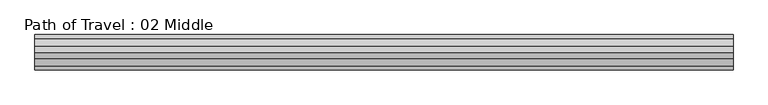
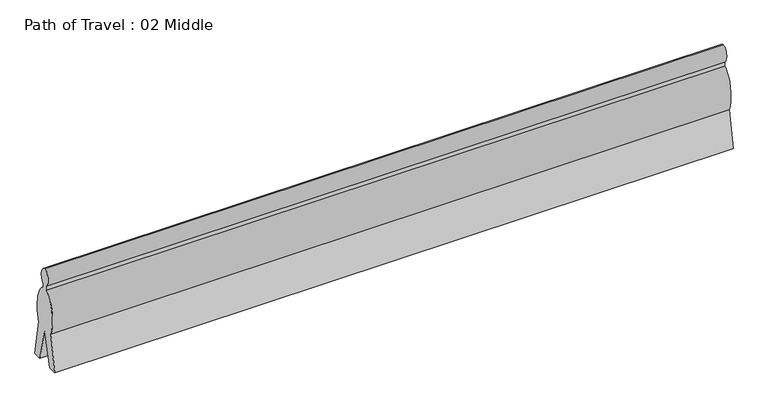
"""IFC4 building model written with IfcOpenShell, lengths in millimetres: proxy geometry, Path of Travel : 02 Middle."""

from ifc_helpers import new_model, si_unit, point, frame, origin, place, context, project, spatial, ellipse_curve, trimmed, source, transform, mapped, element, save
from ifc_brep_helpers import plane_surface, extruded_surface, advanced_brep


def path_of_travel_02_middle_84569f44(model_context):
    return source(origin(), model_context, "Body", "AdvancedBrep", [
        advanced_brep(
        [(227.5554837, 0.0, 1727.2), (227.5554837, 42.9018657, 1436.6534209), (227.5554837, 42.9018657, 1363.4763406), (227.5554837, 184.1186263, 643.4144547), (227.5554837, 297.5699544, 0.0), (227.5554837, 145.6574193, 0.0), (227.5554837, 0.0, 584.2), (227.5554837, -145.6574193, 0.0), (227.5554837, -297.5699544, 0.0), (227.5554837, -184.1186263, 643.4144547), (227.5554837, -42.9018657, 1363.4763406), (227.5554837, -42.9018657, 1436.6534209), (11987.6438615, 0.0, 1727.2), (11987.6438615, -42.9018657, 1436.6534209), (11987.6438615, -42.9018657, 1363.4763406), (11987.6438615, -184.1186263, 643.4144547), (11987.6438615, -297.5699544, 0.0), (11987.6438615, -145.6574193, 0.0), (11987.6438615, 0.0, 584.2), (11987.6438615, 145.6574193, 0.0), (11987.6438615, 297.5699544, 0.0), (11987.6438615, 184.1186263, 643.4144547), (11987.6438615, 42.9018657, 1363.4763406), (11987.6438615, 42.9018657, 1436.6534209)],
        [
            (0, 1, ellipse_curve(frame((227.5554837, 0.0, 1574.8), z_axis=(-1.0, 0.0, 0.0), x_axis=(0.0, 0.0, 1.0)), 152.4, 101.6)),
            (1, 2),
            (2, 3, ellipse_curve(frame((227.5554837, 0.0, 914.4), z_axis=(-1.0, 0.0, 0.0), x_axis=(0.0, 0.0, -1.0)), 457.2, 228.6)),
            (3, 4),
            (4, 5),
            (5, 6),
            (6, 7),
            (7, 8),
            (8, 9),
            (9, 10, ellipse_curve(frame((227.5554837, 0.0, 914.4), z_axis=(-1.0, 0.0, 0.0), x_axis=(0.0, 0.0, -1.0)), 457.2, 228.6)),
            (10, 11),
            (11, 0, ellipse_curve(frame((227.5554837, 0.0, 1574.8), z_axis=(-1.0, 0.0, 0.0), x_axis=(0.0, 0.0, 1.0)), 152.4, 101.6)),
            (12, 13, ellipse_curve(frame((11987.6438615, 0.0, 1574.8), z_axis=(1.0, 0.0, 0.0), x_axis=(0.0, 0.0, 1.0)), 152.4, 101.6)),
            (13, 14),
            (14, 15, ellipse_curve(frame((11987.6438615, 0.0, 914.4), z_axis=(1.0, 0.0, 0.0), x_axis=(0.0, 0.0, -1.0)), 457.2, 228.6)),
            (15, 16),
            (16, 17),
            (17, 18),
            (18, 19),
            (19, 20),
            (20, 21),
            (21, 22, ellipse_curve(frame((11987.6438615, 0.0, 914.4), z_axis=(1.0, 0.0, 0.0), x_axis=(0.0, 0.0, -1.0)), 457.2, 228.6)),
            (22, 23),
            (23, 12, ellipse_curve(frame((11987.6438615, 0.0, 1574.8), z_axis=(1.0, 0.0, 0.0), x_axis=(0.0, 0.0, 1.0)), 152.4, 101.6)),
            (0, 12),
            (23, 1),
            (22, 2),
            (21, 3),
            (20, 4),
            (19, 5),
            (18, 6),
            (17, 7),
            (16, 8),
            (15, 9),
            (14, 10),
            (13, 11),
        ],
        [
            plane_surface(frame((227.5554837, 0.0, 0.0), z_axis=(-1.0, 0.0, 0.0), x_axis=(0.0, 0.0, 1.0))),
            plane_surface(frame((11987.6438615, 0.0, 0.0), z_axis=(1.0, 0.0, 0.0), x_axis=(0.0, 0.0, 1.0))),
            extruded_surface(trimmed(ellipse_curve(frame((11987.6438615, 0.0, 1574.8), z_axis=(-1.0, 0.0, 0.0), x_axis=(0.0, 0.0, 1.0)), 152.4, 101.6), [point((11987.6438615, 0.0, 1727.2))], [point((11987.6438615, 42.9018657, 1436.6534209))], True, "CARTESIAN"), (-11760.0883778, 0.0, 0.0), 11760.0883778),
            plane_surface(frame((227.5554837, 42.9018657, 1436.6534209), z_axis=(0.0, 1.0, 0.0), x_axis=(1.0, 0.0, 0.0))),
            extruded_surface(trimmed(ellipse_curve(frame((11987.6438615, 0.0, 914.4), z_axis=(-1.0, 0.0, 0.0), x_axis=(0.0, 0.0, -1.0)), 457.2, 228.6), [point((11987.6438615, 42.9018657, 1363.4763406))], [point((11987.6438615, 184.1186263, 643.4144547))], True, "CARTESIAN"), (-11760.0883778, 0.0, 0.0), 11760.0883778),
            plane_surface(frame((227.5554837, 184.1186263, 643.4144547), z_axis=(0.0, 0.9848077530122078, 0.17364817766693205), x_axis=(1.0, 0.0, 0.0))),
            plane_surface(frame((227.5554837, 297.5699544, 0.0), z_axis=(0.0, 0.0, -1.0), x_axis=(1.0, 0.0, 0.0))),
            plane_surface(frame((227.5554837, 145.6574193, 0.0), z_axis=(0.0, -0.9702957262760199, -0.2419218955995739), x_axis=(1.0, 0.0, 0.0))),
            plane_surface(frame((227.5554837, 0.0, 584.2), z_axis=(0.0, 0.9702957262759961, -0.24192189559966923), x_axis=(1.0, 0.0, 0.0))),
            plane_surface(frame((227.5554837, -145.6574193, 0.0), z_axis=(0.0, 0.0, -1.0), x_axis=(1.0, 0.0, 0.0))),
            plane_surface(frame((227.5554837, -297.5699544, 0.0), z_axis=(0.0, -0.984807753012208, 0.17364817766693066), x_axis=(1.0, 0.0, 0.0))),
            extruded_surface(trimmed(ellipse_curve(frame((11987.6438615, 0.0, 914.4), z_axis=(-1.0, 0.0, 0.0), x_axis=(0.0, 0.0, -1.0)), 457.2, 228.6), [point((11987.6438615, -184.1186263, 643.4144547))], [point((11987.6438615, -42.9018657, 1363.4763406))], True, "CARTESIAN"), (-11760.0883778, 0.0, 0.0), 11760.0883778),
            plane_surface(frame((227.5554837, -42.9018657, 1363.4763406), z_axis=(0.0, -1.0, 0.0), x_axis=(1.0, 0.0, 0.0))),
            extruded_surface(trimmed(ellipse_curve(frame((11987.6438615, 0.0, 1574.8), z_axis=(-1.0, 0.0, 0.0), x_axis=(0.0, 0.0, 1.0)), 152.4, 101.6), [point((11987.6438615, -42.9018657, 1436.6534209))], [point((11987.6438615, 0.0, 1727.2))], True, "CARTESIAN"), (-11760.0883778, 0.0, 0.0), 11760.0883778),
        ],
        [
            (0, [[1, 2, 3, 4, 5, 6, 7, 8, 9, 10, 11, 12]]),
            (1, [[13, 14, 15, 16, 17, 18, 19, 20, 21, 22, 23, 24]]),
            (2, [[-1, 25, -24, 26]]),
            (3, [[-2, -26, -23, 27]]),
            (4, [[-3, -27, -22, 28]]),
            (5, [[-4, -28, -21, 29]]),
            (6, [[-5, -29, -20, 30]]),
            (7, [[-6, -30, -19, 31]]),
            (8, [[-7, -31, -18, 32]]),
            (9, [[-8, -32, -17, 33]]),
            (10, [[-9, -33, -16, 34]]),
            (11, [[-10, -34, -15, 35]]),
            (12, [[-11, -35, -14, 36]]),
            (13, [[-12, -36, -13, -25]]),
        ],
    ),
    ])


if __name__ == "__main__":
    model = new_model("IFC4")
    model_context = context("Model", 3, world=origin())
    ifc_project = project(units=[si_unit("LENGTHUNIT", "METRE", prefix="MILLI")], contexts=[model_context])
    site = spatial("IfcSite", under=ifc_project)
    building = spatial("IfcBuilding", under=site)
    placement = place(None, origin())
    path_of_travel_02_middle_shape = path_of_travel_02_middle_84569f44(model_context)
    element("IfcBuildingElementProxy", 1, Name="Path of Travel : 02 Middle", ObjectType="Path of Travel : 02 Middle", at=placement, inside=building, context=model_context, shape_type="MappedRepresentation", body=[
        mapped(path_of_travel_02_middle_shape, transform((0.0, 0.0, 0.0), x_axis=(1.0, 0.0, 0.0), y_axis=(0.0, 1.0, 0.0), z_axis=(0.0, 0.0, 1.0))),
    ])
    save(model, "model.ifc")

# Revit data of these elements
# Type "Path of Travel : 02 Middle"
#   Path of Egress [instance default] = 4' - 0"
#   built-in parameter 1001306 [instance default] = 4 (stored number, unit not read)
#   Dot at Start = no
#   Arrow in Middle = yes
#   Arrow at End = no
#   Egress Path = none
# Element 1 (IfcBuildingElementProxy, "Path of Travel : 02 Middle")
#   Path of Egress = 38' - 6.99561"
#   built-in parameter 1001306 = 38.583 (stored number, unit not read)
#   Materials on its faces: "Egress Path Solid"
# Materials
#   "Egress Path Solid": class "Unassigned", colour RGB 255 128 64, transparency 0.75, Comments = "Rendering appearance not upgraded "
